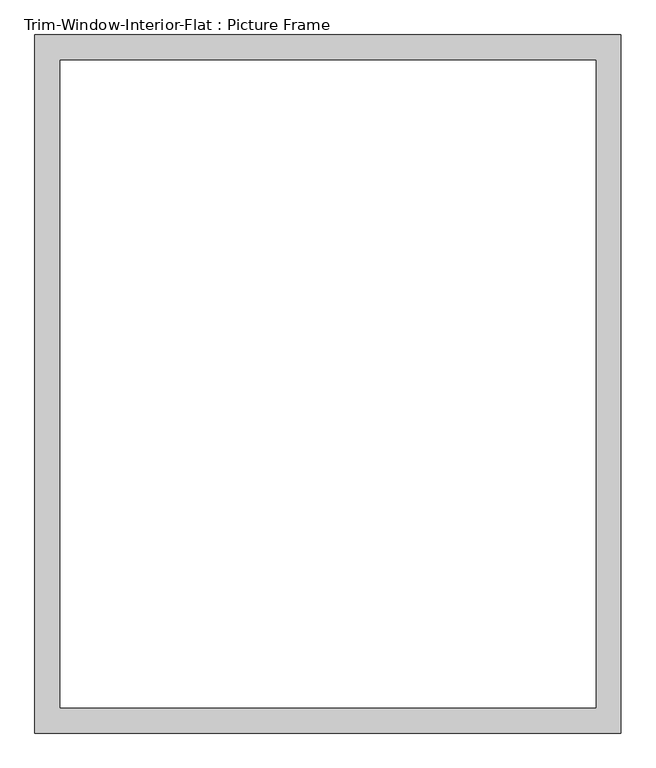
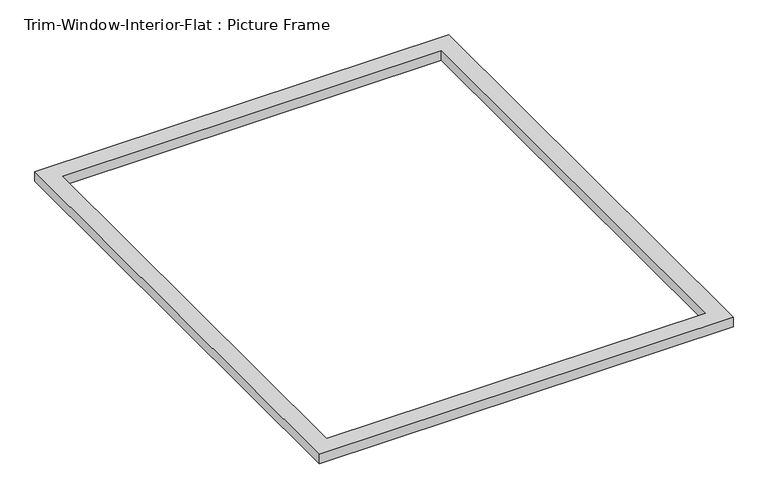
"""IFC4 building model written with IfcOpenShell, lengths in millimetres: proxy geometry, Trim-Window-Interior-Flat : Picture Frame."""

from ifc_helpers import new_model, si_unit, origin, origin_with_axes, place, context, project, spatial, polyline, outline, extrude, source, transform, mapped, element, save


def trim_window_interior_flat_picture_frame_cd30aacc(model_context):
    return source(origin(), model_context, "Body", "SweptSolid", [
        extrude(outline(polyline([(666.75, -44.45), (-666.75, -44.45), (-666.75, 1543.05), (666.75, 1543.05), (666.75, -44.45)]), holes=[polyline([(609.6, 12.7), (609.6, 1485.9), (-609.6, 1485.9), (-609.6, 12.7), (609.6, 12.7)])]), origin_with_axes(), (0.0, 0.0, 1.0), 31.75),
    ])


if __name__ == "__main__":
    model = new_model("IFC4")
    model_context = context("Model", 3, world=origin())
    ifc_project = project(units=[si_unit("LENGTHUNIT", "METRE", prefix="MILLI")], contexts=[model_context])
    site = spatial("IfcSite", under=ifc_project)
    building = spatial("IfcBuilding", under=site)
    placement = place(None, origin())
    trim_window_interior_flat_picture_frame_shape = trim_window_interior_flat_picture_frame_cd30aacc(model_context)
    element("IfcBuildingElementProxy", 1, Name="Trim-Window-Interior-Flat : Picture Frame", ObjectType="Trim-Window-Interior-Flat : Picture Frame", at=placement, inside=building, context=model_context, shape_type="MappedRepresentation", body=[
        mapped(trim_window_interior_flat_picture_frame_shape, transform((0.0, 0.0, 0.0), x_axis=(1.0, 0.0, 0.0), y_axis=(0.0, 1.0, 0.0), z_axis=(0.0, 0.0, 1.0))),
    ])
    save(model, "model.ifc")

# Revit data of these elements
# Type "Trim-Window-Interior-Flat : Picture Frame"
#   Trim Thickness_Picture Frame = 0' - 1 1/4"
#   Trim Width = 0' - 2 1/4"
#   Trim Thickness_with Sill = 0' - 0 3/4"
#   Sill Thickness = 0' - 1 1/4"
#   Opening Width [instance default] = 2' - 0"
#   Opening Height [instance default] = 3' - 0"
#   Default Elevation = 4' - 0"
#   Sill = no
#   Picture Frame = yes
#   Trim Material [instance default] = none
# Element 1 (IfcBuildingElementProxy, "Trim-Window-Interior-Flat : Picture Frame")
#   Opening Width = 4' - 1"
#   Opening Height = 4' - 11"
#   Trim Material = Wood - Stained
#   Materials on its faces: "Wood - Stained"
# Materials
#   "Wood - Stained": class "Wood", colour RGB 224 178 126, transparency 0, Cost = 0
